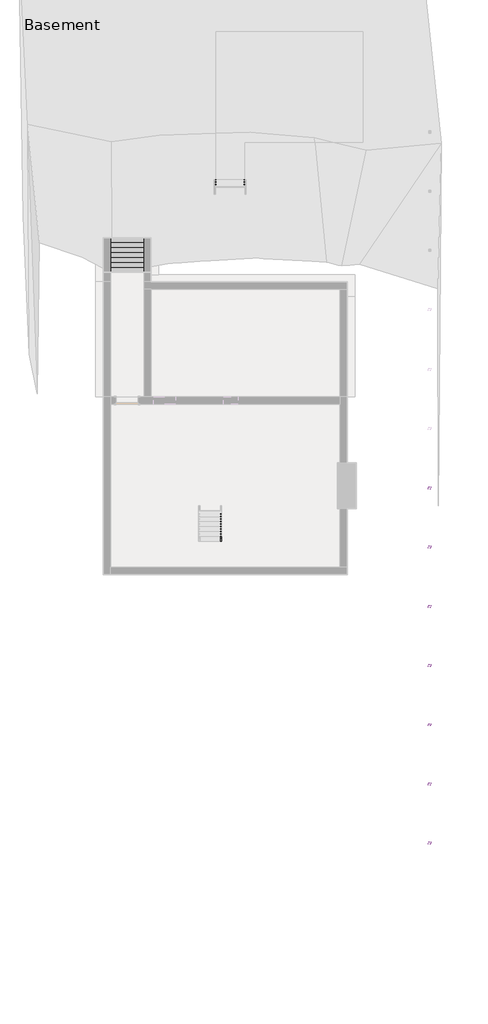
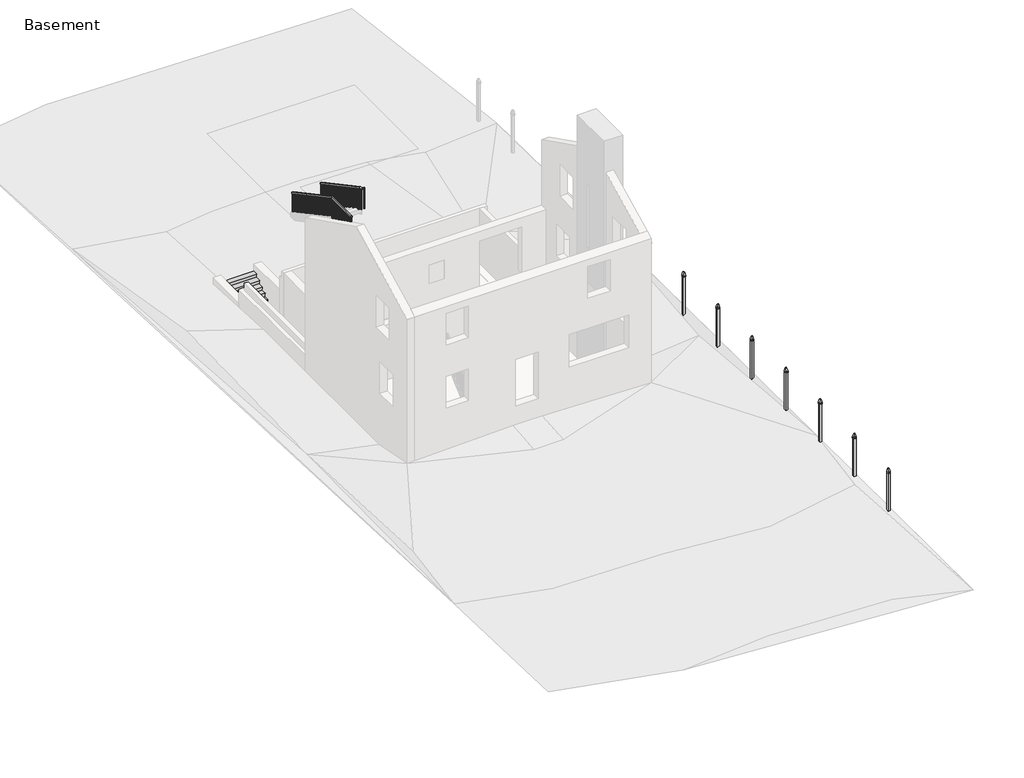
# One storey, part 2 of 3: 7 proxies, 3 railings, 1 stair flight.
"""IFC4 building model written with IfcOpenShell, lengths in millimetres."""

import ifcopenshell
import ifcopenshell.guid

model = None  # the IFC model being written
_history = None  # IfcOwnerHistory: only IFC2X3 demands one
_inside = {}  # id of a spatial element -> (the spatial element, [elements in it])
_under = {}  # id of a project, library or spatial element -> (it, [spatial elements below it])
_declared = {}  # id of a project -> (the project, [libraries it declares])
_typed = {}  # id of a type object -> (the type object, [elements of that type])
_made_of = {}  # id of a material, layer set ... -> (it, [elements and type objects made of it])


def new_model(schema):
    """Start an empty IFC model of exactly this schema.

    Asked for "IFC4X3", IfcOpenShell would pick the latest addendum, in which some entities
    have other attributes; the version numbers below select the first issue.
    IFC2X3 requires an IfcOwnerHistory on every rooted entity: one is made here for all.
    """
    global model, _history
    if schema == "IFC4X3":
        model = ifcopenshell.file(schema_version=(4, 3, 0, 0))
    else:
        model = ifcopenshell.file(schema=schema)
    _inside.clear()
    _under.clear()
    _declared.clear()
    _typed.clear()
    _made_of.clear()
    _history = None
    if model.schema == "IFC2X3":
        org = make("IfcOrganization", Name="unknown")
        user = make(
            "IfcPersonAndOrganization",
            ThePerson=make("IfcPerson", FamilyName="unknown"),
            TheOrganization=org,
        )
        app = make(
            "IfcApplication",
            ApplicationDeveloper=org,
            Version="unknown",
            ApplicationFullName="unknown",
            ApplicationIdentifier="unknown",
        )
        _history = make(
            "IfcOwnerHistory",
            OwningUser=user,
            OwningApplication=app,
            ChangeAction="ADDED",
            CreationDate=0,
        )
    return model


def make(cls, **values):
    """One entity of the class cls with the attributes given. An attribute that is None is left unset."""
    return model.create_entity(
        cls, **{name: value for name, value in values.items() if value is not None}
    )


def rooted(cls, **values):
    """An entity with a GlobalId (a new one), such as an element, a storey or a relation."""
    return make(cls, GlobalId=ifcopenshell.guid.new(), OwnerHistory=_history, **values)


def si_unit(unit_type, name, prefix=None):
    """IfcSIUnit, for example si_unit("LENGTHUNIT", "METRE", prefix="MILLI")."""
    return make("IfcSIUnit", UnitType=unit_type, Prefix=prefix, Name=name)


def assignment(units):
    """IfcUnitAssignment: the units of a project."""
    return None if units is None else make("IfcUnitAssignment", Units=units)


def point(xyz):
    """IfcCartesianPoint."""
    return None if xyz is None else make("IfcCartesianPoint", Coordinates=xyz)


def direction(xyz):
    """IfcDirection."""
    return None if xyz is None else make("IfcDirection", DirectionRatios=xyz)


def frame(location, z_axis=None, x_axis=None):
    """IfcAxis2Placement3D, a coordinate frame: its origin and axes. An axis left out is left unset."""
    return make(
        "IfcAxis2Placement3D",
        Location=point(location),
        Axis=direction(z_axis),
        RefDirection=direction(x_axis),
    )


def origin():
    """The frame at (0, 0, 0) with its axes left unset."""
    return frame((0.0, 0.0, 0.0))


def origin_with_axes():
    """The frame at (0, 0, 0) with the z axis (0, 0, 1) and the x axis (1, 0, 0) written out."""
    return frame((0.0, 0.0, 0.0), z_axis=(0.0, 0.0, 1.0), x_axis=(1.0, 0.0, 0.0))


def place(relative_to, where):
    """IfcLocalPlacement: puts the frame where relative to a parent placement (None: the world)."""
    return make(
        "IfcLocalPlacement", PlacementRelTo=relative_to, RelativePlacement=where
    )


def context(
    kind, dimensions, precision=None, world=None, true_north=None, identifier=None
):
    """IfcGeometricRepresentationContext, for example the 3D "Model" context."""
    return make(
        "IfcGeometricRepresentationContext",
        ContextIdentifier=identifier,
        ContextType=kind,
        CoordinateSpaceDimension=dimensions,
        Precision=precision,
        WorldCoordinateSystem=world,
        TrueNorth=true_north,
    )


def project(units=None, contexts=None):
    """IfcProject with its units and contexts."""
    return rooted(
        "IfcProject",
        Name="project",
        RepresentationContexts=contexts,
        UnitsInContext=assignment(units),
    )


def spatial(cls, under=None, at=None, **own):
    """A site, building, storey or space (cls), placed at a placement, below another one or the project."""
    s = rooted(cls, ObjectPlacement=at, **own)
    if under is not None:
        _under.setdefault(under.id(), (under, []))[1].append(s)
    return s


def polyline(points):
    """IfcPolyline through the points."""
    return make("IfcPolyline", Points=[point(p) for p in points])


def ellipse_curve(where, semi_axis1, semi_axis2):
    """IfcEllipse in the frame where."""
    return make(
        "IfcEllipse", Position=where, SemiAxis1=semi_axis1, SemiAxis2=semi_axis2
    )


def outline(outer, holes=None, kind="AREA"):
    """IfcArbitraryClosedProfileDef: a profile drawn as a closed curve; with holes, ...WithVoids."""
    if holes is None:
        return make("IfcArbitraryClosedProfileDef", ProfileType=kind, OuterCurve=outer)
    return make(
        "IfcArbitraryProfileDefWithVoids",
        ProfileType=kind,
        OuterCurve=outer,
        InnerCurves=holes,
    )


def extrude(swept, where, along, depth):
    """IfcExtrudedAreaSolid: the profile swept, set in the frame where, extruded along a direction by depth."""
    return make(
        "IfcExtrudedAreaSolid",
        SweptArea=swept,
        Position=where,
        ExtrudedDirection=direction(along),
        Depth=depth,
    )


def faces_of(points, faces, orient=None, outer=None):
    """IfcFace entities. A face is a list of loops; a loop is a list of indices into points, from 0.

    orient and outer hold one flag for each loop. By default every Orientation is true, the
    first loop of a face is its IfcFaceOuterBound and the others are IfcFaceBound.
    """
    made = []
    for i, loops in enumerate(faces):
        bounds = []
        for j, loop in enumerate(loops):
            is_outer = j == 0 if outer is None else outer[i][j]
            bounds.append(
                make(
                    "IfcFaceOuterBound" if is_outer else "IfcFaceBound",
                    Bound=make("IfcPolyLoop", Polygon=[points[k] for k in loop]),
                    Orientation=True if orient is None else orient[i][j],
                )
            )
        made.append(make("IfcFace", Bounds=bounds))
    return made


def faceted_brep(points, faces, orient=None, outer=None, voids=None):
    """IfcFacetedBrep: a solid bounded by flat faces; with voids (closed shells), ...WithVoids."""
    shared = [point(p) for p in points]
    hull = make("IfcClosedShell", CfsFaces=faces_of(shared, faces, orient, outer))
    if voids is None:
        return make("IfcFacetedBrep", Outer=hull)
    return make(
        "IfcFacetedBrepWithVoids",
        Outer=hull,
        Voids=[
            make(cls, CfsFaces=faces_of(shared, fs, o, b)) for cls, fs, o, b in voids
        ],
    )


def shape(context_of_items, identifier, shape_type, items):
    """IfcShapeRepresentation: the items that make up one representation, for example the "Body"."""
    return make(
        "IfcShapeRepresentation",
        ContextOfItems=context_of_items,
        RepresentationIdentifier=identifier,
        RepresentationType=shape_type,
        Items=items,
    )


def source(mapping_origin, context_of_items, identifier, shape_type, items):
    """IfcRepresentationMap: a shape defined once, which mapped items show again and again."""
    return make(
        "IfcRepresentationMap",
        MappingOrigin=mapping_origin,
        MappedRepresentation=shape(context_of_items, identifier, shape_type, items),
    )


def transform(
    local_origin,
    x_axis=None,
    y_axis=None,
    z_axis=None,
    scale=None,
    scale2=None,
    scale3=None,
    uniform=True,
):
    """IfcCartesianTransformationOperator3D, or its non-uniform kind. x_axis, y_axis, z_axis: its Axis1, 2, 3."""
    if uniform:
        return make(
            "IfcCartesianTransformationOperator3D",
            Axis1=direction(x_axis),
            Axis2=direction(y_axis),
            LocalOrigin=point(local_origin),
            Scale=scale,
            Axis3=direction(z_axis),
        )
    return make(
        "IfcCartesianTransformationOperator3DnonUniform",
        Axis1=direction(x_axis),
        Axis2=direction(y_axis),
        LocalOrigin=point(local_origin),
        Scale=scale,
        Axis3=direction(z_axis),
        Scale2=scale2,
        Scale3=scale3,
    )


def mapped(mapping_source, mapping_target):
    """IfcMappedItem: shows the shape of a source again, moved by a transform."""
    return make(
        "IfcMappedItem", MappingSource=mapping_source, MappingTarget=mapping_target
    )


def made_of(thing, what):
    """Note that an element or type object is made of a material, layer set ...; save() writes the relation."""
    if what is not None:
        _made_of.setdefault(what.id(), (what, []))[1].append(thing)
    return thing


def element(
    cls,
    number,
    at=None,
    inside=None,
    cuts=None,
    type_object=None,
    material=None,
    context=None,
    identifier="Body",
    shape_type=None,
    held_by="IfcProductDefinitionShape",
    body=None,
    shapes=None,
    **own,
):
    """One element of the class cls, such as IfcWall. Its Tag is "e" and its number.

    at: its placement. inside: the storey or other place that contains it. cuts: it is an
    opening in that element (IfcRelVoidsElement). A single representation is given by context,
    identifier, shape_type and body (its items); several are given by shapes. held_by: the class
    of the entity that holds the representations. save() writes the other relations.
    """
    e = rooted(cls, Tag="e%d" % number, ObjectPlacement=at, **own)
    if body is not None:
        shapes = [shape(context, identifier, shape_type, body)]
    if shapes is not None:
        e.Representation = make(held_by, Representations=shapes)
    if inside is not None:
        _inside.setdefault(inside.id(), (inside, []))[1].append(e)
    if cuts is not None:
        rooted(
            "IfcRelVoidsElement", RelatingBuildingElement=cuts, RelatedOpeningElement=e
        )
    if type_object is not None:
        _typed.setdefault(type_object.id(), (type_object, []))[1].append(e)
    return made_of(e, material)


def aggregate(whole, parts):
    """IfcRelAggregates: a whole, such as a stair, and the parts it consists of."""
    return rooted("IfcRelAggregates", RelatingObject=whole, RelatedObjects=parts)


def save(model, path):
    """Write the relations noted so far, then the file.

    IfcRelAggregates (storeys below a building ...), IfcRelContainedInSpatialStructure (elements
    in a storey), IfcRelDefinesByType, IfcRelAssociatesMaterial and IfcRelDeclares: one each for
    every whole, place, type object, material and project.
    """
    for whole, parts in _under.values():
        aggregate(whole, parts)
    for where, things in _inside.values():
        rooted(
            "IfcRelContainedInSpatialStructure",
            RelatedElements=things,
            RelatingStructure=where,
        )
    for kind, things in _typed.values():
        rooted("IfcRelDefinesByType", RelatedObjects=things, RelatingType=kind)
    for what, things in _made_of.values():
        rooted("IfcRelAssociatesMaterial", RelatedObjects=things, RelatingMaterial=what)
    for by, libraries in _declared.values():
        rooted("IfcRelDeclares", RelatingContext=by, RelatedDefinitions=libraries)
    model.write(path)


def plane_surface(at):
    """IfcPlane: the flat surface through the origin of the frame at, square to its z axis."""
    return make("IfcPlane", Position=at)


def cylinder_surface(at, radius):
    """IfcCylindricalSurface: all points at the distance radius from the z axis of the frame at."""
    return make("IfcCylindricalSurface", Position=at, Radius=radius)


def revolved_surface(curve, axis_point, axis_direction):
    """IfcSurfaceOfRevolution: the curve turned about the line through axis_point along axis_direction."""
    return make(
        "IfcSurfaceOfRevolution",
        SweptCurve=make("IfcArbitraryOpenProfileDef", ProfileType="CURVE", Curve=curve),
        AxisPosition=make("IfcAxis1Placement", Location=point(axis_point), Axis=direction(axis_direction)),
    )


def advanced_brep(points, edges, surfaces, faces):
    """IfcAdvancedBrep: a solid bounded by faces that lie on surfaces and meet in shared edges.

    An edge is (start, end): straight between two places in points (the first is 0);
    or (start, end, curve); or (start, end, curve, False) where it runs against its curve.
    A face is (place in surfaces, loops), or (place, loops, False) where it looks against
    its surface's normal. A loop lists edges by number (the first is 1), with a minus sign
    where the edge is run from its end to its start. The first loop is the outer one.
    """
    corners = [point(p) for p in points]
    vertices = [make("IfcVertexPoint", VertexGeometry=c) for c in corners]
    made = []
    for start, end, *more in edges:
        made.append(
            make(
                "IfcEdgeCurve",
                EdgeStart=vertices[start],
                EdgeEnd=vertices[end],
                EdgeGeometry=more[0] if more else make("IfcPolyline", Points=[corners[start], corners[end]]),
                SameSense=more[1] if len(more) > 1 else True,
            )
        )
    hull = []
    for where, loops, *sense in faces:
        bounds = []
        for j, loop in enumerate(loops):
            ring = [make("IfcOrientedEdge", EdgeElement=made[abs(k) - 1], Orientation=k > 0) for k in loop]
            bounds.append(
                make(
                    "IfcFaceOuterBound" if j == 0 else "IfcFaceBound",
                    Bound=make("IfcEdgeLoop", EdgeList=ring),
                    Orientation=True,
                )
            )
        hull.append(make("IfcAdvancedFace", Bounds=bounds, FaceSurface=surfaces[where], SameSense=sense[0] if sense else True))
    return make("IfcAdvancedBrep", Outer=make("IfcClosedShell", CfsFaces=hull))


def proxy_fa72a640(model_context):
    return source(origin(), model_context, "Body", "SolidModel", [
        extrude(outline(polyline([(44.45, 107.95), (44.45, 19.05), (-44.45, 19.05), (-44.45, 107.95), (44.45, 107.95)])), frame((0.0, 0.0, -228.6), z_axis=(0.0, 0.0, 1.0), x_axis=(1.0, 0.0, 0.0)), (0.0, 0.0, 1.0), 1676.4),
        advanced_brep(
        [(44.45, 19.05, 1428.75), (44.45, 19.05, 1447.8), (44.45, 107.95, 1447.8), (44.45, 107.95, 1428.75), (50.8, 12.7, 1460.5), (50.8, 12.7, 1428.75), (50.8, 114.3, 1428.75), (50.8, 114.3, 1460.5), (-44.45, 107.95, 1447.8), (-44.45, 107.95, 1428.75), (-50.8, 114.3, 1428.75), (-50.8, 114.3, 1460.5), (-44.45, 19.05, 1447.8), (-44.45, 19.05, 1428.75), (-50.8, 12.7, 1428.75), (-50.8, 12.7, 1460.5), (21.7547368, 85.2547368, 1622.5472198), (-21.7547368, 85.2547368, 1622.5472198), (-21.7547368, 41.7452632, 1622.5472198), (21.7547368, 41.7452632, 1622.5472198), (50.8, 114.3, 1485.9), (50.8, 12.7, 1485.9), (-50.8, 114.3, 1485.9), (-50.8, 12.7, 1485.9)],
        [
            (0, 1),
            (1, 2),
            (2, 3),
            (3, 0),
            (4, 5),
            (5, 6),
            (6, 7),
            (7, 4),
            (2, 8),
            (8, 9),
            (9, 3),
            (6, 10),
            (10, 11),
            (11, 7),
            (8, 12),
            (12, 13),
            (13, 9),
            (10, 14),
            (14, 15),
            (15, 11),
            (0, 13),
            (12, 1),
            (5, 14),
            (4, 15),
            (16, 17),
            (17, 18),
            (18, 19),
            (19, 16),
            (7, 20, ellipse_curve(frame((57.3454302, 120.8454302, 1473.2), z_axis=(-0.7071067811865475, 0.7071067811865475, 0.0), x_axis=(0.7071067811865474, 0.7071067811865476, 0.0)), 20.2055763, 14.2875)),
            (20, 21),
            (21, 4, ellipse_curve(frame((57.3454302, 6.1545698, 1473.2), z_axis=(-0.7071067811865475, -0.7071067811865475, 0.0), x_axis=(-0.7071067811865474, 0.7071067811865476, 0.0)), 20.2055763, 14.2875)),
            (19, 21, ellipse_curve(frame((-351.3440328, 414.8440328, 1471.8321377), z_axis=(0.7071067811865475, 0.7071067811865475, 0.0), x_axis=(0.7071067811865474, -0.7071067811865476, 0.0)), 569.065423, 402.3900195)),
            (20, 16, ellipse_curve(frame((-351.3440328, -287.8440328, 1471.8321377), z_axis=(0.7071067811865475, -0.7071067811865475, 0.0), x_axis=(-0.7071067811865474, -0.7071067811865476, 0.0)), 569.065423, 402.3900195)),
            (11, 22, ellipse_curve(frame((-57.3454302, 120.8454302, 1473.2), z_axis=(-0.7071067811865475, -0.7071067811865475, 0.0), x_axis=(-0.7071067811865476, 0.7071067811865474, 0.0)), 20.2055763, 14.2875)),
            (22, 20),
            (22, 17, ellipse_curve(frame((351.3440328, -287.8440328, 1471.8321377), z_axis=(0.7071067811865475, 0.7071067811865475, 0.0), x_axis=(0.7071067811865476, -0.7071067811865474, 0.0)), 569.065423, 402.3900195)),
            (15, 23, ellipse_curve(frame((-57.3454302, 6.1545698, 1473.2), z_axis=(0.7071067811865475, -0.7071067811865475, 0.0), x_axis=(-0.7071067811865474, -0.7071067811865476, 0.0)), 20.2055763, 14.2875)),
            (23, 22),
            (23, 18, ellipse_curve(frame((351.3440328, 414.8440328, 1471.8321377), z_axis=(-0.7071067811865475, 0.7071067811865475, 0.0), x_axis=(0.7071067811865474, 0.7071067811865476, 0.0)), 569.065423, 402.3900195)),
            (21, 23),
        ],
        [
            plane_surface(frame((44.45, 19.05, 1447.8), z_axis=(-1.0, 0.0, 0.0), x_axis=(0.0, 1.0, 0.0))),
            plane_surface(frame((50.8, 12.7, 1428.75), z_axis=(1.0, 0.0, 0.0), x_axis=(0.0, 1.0, 0.0))),
            plane_surface(frame((44.45, 107.95, 1447.8), z_axis=(0.0, -1.0, 0.0), x_axis=(-1.0, 0.0, 0.0))),
            plane_surface(frame((50.8, 114.3, 1428.75), z_axis=(0.0, 1.0, 0.0), x_axis=(-1.0, 0.0, 0.0))),
            plane_surface(frame((-44.45, 107.95, 1447.8), z_axis=(1.0, 0.0, 0.0), x_axis=(0.0, -1.0, 0.0))),
            plane_surface(frame((-50.8, 114.3, 1428.75), z_axis=(-1.0, 0.0, 0.0), x_axis=(0.0, -1.0, 0.0))),
            plane_surface(frame((-44.45, 19.05, 1447.8), z_axis=(0.0, 1.0, 0.0), x_axis=(1.0, 0.0, 0.0))),
            plane_surface(frame((-15.4047368, 48.0952632, 1447.8), z_axis=(0.0, 0.0, -1.0), x_axis=(1.0, 0.0, 0.0))),
            plane_surface(frame((-44.45, 19.05, 1428.75), z_axis=(0.0, 0.0, -1.0), x_axis=(1.0, 0.0, 0.0))),
            plane_surface(frame((-50.8, 12.7, 1428.75), z_axis=(0.0, -1.0, 0.0), x_axis=(1.0, 0.0, 0.0))),
            plane_surface(frame((-21.7547368, 41.7452632, 1622.5472198), z_axis=(0.0, 0.0, 1.0), x_axis=(1.0, 0.0, 0.0))),
            revolved_surface(polyline([(43.0579302, 135.1329302195122, 1473.2), (43.0579302, -8.132930219512193, 1473.2)]), (57.3454302, 19.05, 1473.2), (0.0, 1.0, 0.0)),
            cylinder_surface(frame((-351.3440328, 19.05, 1471.8321377), z_axis=(0.0, -1.0, 0.0), x_axis=(-1.0, 0.0, 0.0)), 402.3900195),
            revolved_surface(polyline([(-71.63293021951219, 106.5579302, 1473.2), (71.63293021951219, 106.5579302, 1473.2)]), (44.45, 120.8454302, 1473.2), (-1.0, 0.0, 0.0)),
            cylinder_surface(frame((44.45, -287.8440328, 1471.8321377), z_axis=(1.0, 0.0, 0.0), x_axis=(0.0, -1.0, 0.0)), 402.3900195),
            revolved_surface(polyline([(-43.0579302, -8.13293021951219, 1473.2), (-43.0579302, 135.1329302195122, 1473.2)]), (-57.3454302, 107.95, 1473.2), (0.0, -1.0, 0.0)),
            cylinder_surface(frame((351.3440328, 107.95, 1471.8321377), z_axis=(0.0, 1.0, 0.0), x_axis=(1.0, 0.0, 0.0)), 402.3900195),
            revolved_surface(polyline([(71.63293021951218, 20.4420698, 1473.2), (-71.63293021951219, 20.4420698, 1473.2)]), (-44.45, 6.1545698, 1473.2), (1.0, 0.0, 0.0)),
            cylinder_surface(frame((-44.45, 414.8440328, 1471.8321377), z_axis=(-1.0, 0.0, 0.0), x_axis=(0.0, 1.0, 0.0)), 402.3900195),
        ],
        [
            (0, [[1, 2, 3, 4]]),
            (1, [[5, 6, 7, 8]]),
            (2, [[-3, 9, 10, 11]]),
            (3, [[-7, 12, 13, 14]]),
            (4, [[-10, 15, 16, 17]]),
            (5, [[-13, 18, 19, 20]]),
            (6, [[-1, 21, -16, 22]]),
            (7, [[-2, -22, -15, -9]]),
            (8, [[-6, 23, -18, -12], [-4, -11, -17, -21]]),
            (9, [[-5, 24, -19, -23]]),
            (10, [[25, 26, 27, 28]]),
            (11, [[-8, 29, 30, 31]]),
            (12, [[-28, 32, -30, 33]]),
            (13, [[-14, 34, 35, -29]]),
            (14, [[-25, -33, -35, 36]]),
            (15, [[-20, 37, 38, -34]]),
            (16, [[-26, -36, -38, 39]]),
            (17, [[-24, -31, 40, -37]]),
            (18, [[-27, -39, -40, -32]]),
        ],
    ),
    ])


model = new_model("IFC4")

# Units and contexts
model_context = context("Model", 3, world=origin())
ifc_project = project(units=[si_unit("LENGTHUNIT", "METRE", prefix="MILLI")], contexts=[model_context])

# Site, building, storey
site = spatial("IfcSite", under=ifc_project)
building = spatial("IfcBuilding", under=site)
storey = spatial("IfcBuildingStorey", under=building, Name="Basement", Elevation=-2667.0)

# Proxies
placement = place(None, origin())
proxy_shape = proxy_fa72a640(model_context)
element("IfcBuildingElementProxy", 1, Name="SUP_Post : 4\" x 4\"", ObjectType="SUP_Post : 4\" x 4\"", at=placement, inside=storey, context=model_context, shape_type="MappedRepresentation", body=[
    mapped(proxy_shape, transform((7523.8891925, -597.8195486, -1086.34775), x_axis=(0.0, 1.0, 0.0), y_axis=(-1.0, 0.0, 0.0), z_axis=(0.0, 0.0, 1.0))),
])
element("IfcBuildingElementProxy", 2, Name="SUP_Post : 4\" x 4\"", ObjectType="SUP_Post : 4\" x 4\"", at=placement, inside=storey, context=model_context, shape_type="MappedRepresentation", body=[
    mapped(proxy_shape, transform((7523.8891925, -3034.8101148, -1003.4529933), x_axis=(0.0, 1.0, 0.0), y_axis=(-1.0, 0.0, 0.0), z_axis=(0.0, 0.0, 1.0))),
])
element("IfcBuildingElementProxy", 3, Name="SUP_Post : 4\" x 4\"", ObjectType="SUP_Post : 4\" x 4\"", at=placement, inside=storey, context=model_context, shape_type="MappedRepresentation", body=[
    mapped(proxy_shape, transform((7523.8891925, -5471.8006809, -920.5582365), x_axis=(0.0, 1.0, 0.0), y_axis=(-1.0, 0.0, 0.0), z_axis=(0.0, 0.0, 1.0))),
])
element("IfcBuildingElementProxy", 4, Name="SUP_Post : 4\" x 4\"", ObjectType="SUP_Post : 4\" x 4\"", at=placement, inside=storey, context=model_context, shape_type="MappedRepresentation", body=[
    mapped(proxy_shape, transform((7523.8891925, -7908.3149466, -826.7906503), x_axis=(0.0, 1.0, 0.0), y_axis=(-1.0, 0.0, 0.0), z_axis=(0.0, 0.0, 1.0))),
])
element("IfcBuildingElementProxy", 5, Name="SUP_Post : 4\" x 4\"", ObjectType="SUP_Post : 4\" x 4\"", at=placement, inside=storey, context=model_context, shape_type="MappedRepresentation", body=[
    mapped(proxy_shape, transform((7523.8891925, -10343.9591395, -723.8999758), x_axis=(0.0, 1.0, 0.0), y_axis=(-1.0, 0.0, 0.0), z_axis=(0.0, 0.0, 1.0))),
])
element("IfcBuildingElementProxy", 6, Name="SUP_Post : 4\" x 4\"", ObjectType="SUP_Post : 4\" x 4\"", at=placement, inside=storey, context=model_context, shape_type="MappedRepresentation", body=[
    mapped(proxy_shape, transform((7523.8891925, -12782.1972588, -749.7426083), x_axis=(0.0, 1.0, 0.0), y_axis=(-1.0, 0.0, 0.0), z_axis=(0.0, 0.0, 1.0))),
])
element("IfcBuildingElementProxy", 7, Name="SUP_Post : 4\" x 4\"", ObjectType="SUP_Post : 4\" x 4\"", at=placement, inside=storey, context=model_context, shape_type="MappedRepresentation", body=[
    mapped(proxy_shape, transform((7523.8891925, -15220.4059061, -780.2901471), x_axis=(0.0, 1.0, 0.0), y_axis=(-1.0, 0.0, 0.0), z_axis=(0.0, 0.0, 1.0))),
])

# Railings
element("IfcRailing", 8, ObjectType="Handrail - Rectangular", at=placement, inside=storey, context=model_context, shape_type="SweptSolid", body=[
    extrude(outline(polyline([(-2791.5111242, -1631.7331862), (-2791.5111242, -1562.1), (-149.9111242, 914.4), (-149.9111242, 844.7668138), (-2791.5111242, -1631.7331862)])), frame((-1163.1803068, 0.0, 0.0), z_axis=(1.0, 0.0, 0.0), x_axis=(0.0, 1.0, 0.0)), (0.0, 0.0, 1.0), 50.8),
    extrude(outline(polyline([(-261.0361242, 740.5871263), (-241.9861242, 758.4465013), (-241.9861242, -190.5), (-261.0361242, -190.5), (-261.0361242, 740.5871263)])), frame((-1147.3053068, 0.0, 0.0), z_axis=(1.0, 0.0, 0.0), x_axis=(0.0, 1.0, 0.0)), (0.0, 0.0, 1.0), 19.05),
    extrude(outline(polyline([(-362.6361242, 645.3371263), (-343.5861242, 663.1965013), (-343.5861242, -190.5), (-362.6361242, -190.5), (-362.6361242, 645.3371263)])), frame((-1147.3053068, 0.0, 0.0), z_axis=(1.0, 0.0, 0.0), x_axis=(0.0, 1.0, 0.0)), (0.0, 0.0, 1.0), 19.05),
    extrude(outline(polyline([(-464.2361242, 550.0871263), (-445.1861242, 567.9465013), (-445.1861242, -381.0), (-464.2361242, -381.0), (-464.2361242, 550.0871263)])), frame((-1147.3053068, 0.0, 0.0), z_axis=(1.0, 0.0, 0.0), x_axis=(0.0, 1.0, 0.0)), (0.0, 0.0, 1.0), 19.05),
    extrude(outline(polyline([(-565.8361242, 454.8371263), (-546.7861242, 472.6965013), (-546.7861242, -381.0), (-565.8361242, -381.0), (-565.8361242, 454.8371263)])), frame((-1147.3053068, 0.0, 0.0), z_axis=(1.0, 0.0, 0.0), x_axis=(0.0, 1.0, 0.0)), (0.0, 0.0, 1.0), 19.05),
    extrude(outline(polyline([(-667.4361242, 359.5871263), (-648.3861242, 377.4465013), (-648.3861242, -571.5), (-667.4361242, -571.5), (-667.4361242, 359.5871263)])), frame((-1147.3053068, 0.0, 0.0), z_axis=(1.0, 0.0, 0.0), x_axis=(0.0, 1.0, 0.0)), (0.0, 0.0, 1.0), 19.05),
    extrude(outline(polyline([(-769.0361242, 264.3371263), (-749.9861242, 282.1965013), (-749.9861242, -571.5), (-769.0361242, -571.5), (-769.0361242, 264.3371263)])), frame((-1147.3053068, 0.0, 0.0), z_axis=(1.0, 0.0, 0.0), x_axis=(0.0, 1.0, 0.0)), (0.0, 0.0, 1.0), 19.05),
    extrude(outline(polyline([(-870.6361242, 169.0871263), (-851.5861242, 186.9465013), (-851.5861242, -762.0), (-870.6361242, -762.0), (-870.6361242, 169.0871263)])), frame((-1147.3053068, 0.0, 0.0), z_axis=(1.0, 0.0, 0.0), x_axis=(0.0, 1.0, 0.0)), (0.0, 0.0, 1.0), 19.05),
    extrude(outline(polyline([(-972.2361242, 73.8371263), (-953.1861242, 91.6965013), (-953.1861242, -762.0), (-972.2361242, -762.0), (-972.2361242, 73.8371263)])), frame((-1147.3053068, 0.0, 0.0), z_axis=(1.0, 0.0, 0.0), x_axis=(0.0, 1.0, 0.0)), (0.0, 0.0, 1.0), 19.05),
    extrude(outline(polyline([(-1073.8361242, -21.4128737), (-1054.7861242, -3.5534987), (-1054.7861242, -952.5), (-1073.8361242, -952.5), (-1073.8361242, -21.4128737)])), frame((-1147.3053068, 0.0, 0.0), z_axis=(1.0, 0.0, 0.0), x_axis=(0.0, 1.0, 0.0)), (0.0, 0.0, 1.0), 19.05),
    extrude(outline(polyline([(-1175.4361242, -116.6628737), (-1156.3861242, -98.8034987), (-1156.3861242, -952.5), (-1175.4361242, -952.5), (-1175.4361242, -116.6628737)])), frame((-1147.3053068, 0.0, 0.0), z_axis=(1.0, 0.0, 0.0), x_axis=(0.0, 1.0, 0.0)), (0.0, 0.0, 1.0), 19.05),
    extrude(outline(polyline([(-1277.0361242, -211.9128737), (-1257.9861242, -194.0534987), (-1257.9861242, -1143.0), (-1277.0361242, -1143.0), (-1277.0361242, -211.9128737)])), frame((-1147.3053068, 0.0, 0.0), z_axis=(1.0, 0.0, 0.0), x_axis=(0.0, 1.0, 0.0)), (0.0, 0.0, 1.0), 19.05),
    extrude(outline(polyline([(-1378.6361242, -307.1628737), (-1359.5861242, -289.3034987), (-1359.5861242, -1143.0), (-1378.6361242, -1143.0), (-1378.6361242, -307.1628737)])), frame((-1147.3053068, 0.0, 0.0), z_axis=(1.0, 0.0, 0.0), x_axis=(0.0, 1.0, 0.0)), (0.0, 0.0, 1.0), 19.05),
    extrude(outline(polyline([(-1480.2361242, -402.4128737), (-1461.1861242, -384.5534987), (-1461.1861242, -1333.5), (-1480.2361242, -1333.5), (-1480.2361242, -402.4128737)])), frame((-1147.3053068, 0.0, 0.0), z_axis=(1.0, 0.0, 0.0), x_axis=(0.0, 1.0, 0.0)), (0.0, 0.0, 1.0), 19.05),
    extrude(outline(polyline([(-1581.8361242, -497.6628737), (-1562.7861242, -479.8034987), (-1562.7861242, -1333.5), (-1581.8361242, -1333.5), (-1581.8361242, -497.6628737)])), frame((-1147.3053068, 0.0, 0.0), z_axis=(1.0, 0.0, 0.0), x_axis=(0.0, 1.0, 0.0)), (0.0, 0.0, 1.0), 19.05),
    extrude(outline(polyline([(-1683.4361242, -592.9128737), (-1664.3861242, -575.0534987), (-1664.3861242, -1524.0), (-1683.4361242, -1524.0), (-1683.4361242, -592.9128737)])), frame((-1147.3053068, 0.0, 0.0), z_axis=(1.0, 0.0, 0.0), x_axis=(0.0, 1.0, 0.0)), (0.0, 0.0, 1.0), 19.05),
    extrude(outline(polyline([(-1785.0361242, -688.1628737), (-1765.9861242, -670.3034987), (-1765.9861242, -1524.0), (-1785.0361242, -1524.0), (-1785.0361242, -688.1628737)])), frame((-1147.3053068, 0.0, 0.0), z_axis=(1.0, 0.0, 0.0), x_axis=(0.0, 1.0, 0.0)), (0.0, 0.0, 1.0), 19.05),
    extrude(outline(polyline([(-1886.6361242, -783.4128737), (-1867.5861242, -765.5534987), (-1867.5861242, -1714.5), (-1886.6361242, -1714.5), (-1886.6361242, -783.4128737)])), frame((-1147.3053068, 0.0, 0.0), z_axis=(1.0, 0.0, 0.0), x_axis=(0.0, 1.0, 0.0)), (0.0, 0.0, 1.0), 19.05),
    extrude(outline(polyline([(-1988.2361242, -878.6628737), (-1969.1861242, -860.8034987), (-1969.1861242, -1714.5), (-1988.2361242, -1714.5), (-1988.2361242, -878.6628737)])), frame((-1147.3053068, 0.0, 0.0), z_axis=(1.0, 0.0, 0.0), x_axis=(0.0, 1.0, 0.0)), (0.0, 0.0, 1.0), 19.05),
    extrude(outline(polyline([(-2089.8361242, -973.9128737), (-2070.7861242, -956.0534987), (-2070.7861242, -1905.0), (-2089.8361242, -1905.0), (-2089.8361242, -973.9128737)])), frame((-1147.3053068, 0.0, 0.0), z_axis=(1.0, 0.0, 0.0), x_axis=(0.0, 1.0, 0.0)), (0.0, 0.0, 1.0), 19.05),
    extrude(outline(polyline([(-2191.4361242, -1069.1628737), (-2172.3861242, -1051.3034987), (-2172.3861242, -1905.0), (-2191.4361242, -1905.0), (-2191.4361242, -1069.1628737)])), frame((-1147.3053068, 0.0, 0.0), z_axis=(1.0, 0.0, 0.0), x_axis=(0.0, 1.0, 0.0)), (0.0, 0.0, 1.0), 19.05),
    extrude(outline(polyline([(-2293.0361242, -1164.4128737), (-2273.9861242, -1146.5534987), (-2273.9861242, -2095.5), (-2293.0361242, -2095.5), (-2293.0361242, -1164.4128737)])), frame((-1147.3053068, 0.0, 0.0), z_axis=(1.0, 0.0, 0.0), x_axis=(0.0, 1.0, 0.0)), (0.0, 0.0, 1.0), 19.05),
    extrude(outline(polyline([(-2394.6361242, -1259.6628737), (-2375.5861242, -1241.8034987), (-2375.5861242, -2095.5), (-2394.6361242, -2095.5), (-2394.6361242, -1259.6628737)])), frame((-1147.3053068, 0.0, 0.0), z_axis=(1.0, 0.0, 0.0), x_axis=(0.0, 1.0, 0.0)), (0.0, 0.0, 1.0), 19.05),
    extrude(outline(polyline([(-2496.2361242, -1354.9128737), (-2477.1861242, -1337.0534987), (-2477.1861242, -2286.0), (-2496.2361242, -2286.0), (-2496.2361242, -1354.9128737)])), frame((-1147.3053068, 0.0, 0.0), z_axis=(1.0, 0.0, 0.0), x_axis=(0.0, 1.0, 0.0)), (0.0, 0.0, 1.0), 19.05),
    extrude(outline(polyline([(-2597.8361242, -1450.1628737), (-2578.7861242, -1432.3034987), (-2578.7861242, -2286.0), (-2597.8361242, -2286.0), (-2597.8361242, -1450.1628737)])), frame((-1147.3053068, 0.0, 0.0), z_axis=(1.0, 0.0, 0.0), x_axis=(0.0, 1.0, 0.0)), (0.0, 0.0, 1.0), 19.05),
    extrude(outline(polyline([(-2699.4361242, -1545.4128737), (-2680.3861242, -1527.5534987), (-2680.3861242, -2476.5), (-2699.4361242, -2476.5), (-2699.4361242, -1545.4128737)])), frame((-1147.3053068, 0.0, 0.0), z_axis=(1.0, 0.0, 0.0), x_axis=(0.0, 1.0, 0.0)), (0.0, 0.0, 1.0), 19.05),
    extrude(outline(polyline([(-168.9611242, 826.9074388), (-149.9111242, 844.7668138), (-149.9111242, -190.5), (-168.9611242, -190.5), (-168.9611242, 826.9074388)])), frame((-1147.3053068, 0.0, 0.0), z_axis=(1.0, 0.0, 0.0), x_axis=(0.0, 1.0, 0.0)), (0.0, 0.0, 1.0), 19.05),
    extrude(outline(polyline([(-2791.5111242, -1631.7331862), (-2772.4611242, -1613.8738112), (-2772.4611242, -2476.5), (-2791.5111242, -2476.5), (-2791.5111242, -1631.7331862)])), frame((-1147.3053068, 0.0, 0.0), z_axis=(1.0, 0.0, 0.0), x_axis=(0.0, 1.0, 0.0)), (0.0, 0.0, 1.0), 19.05),
])
element("IfcRailing", 9, ObjectType="Handrail - Rectangular", at=placement, inside=storey, context=model_context, shape_type="SolidModel", body=[
    faceted_brep([(-1315.5803068, 12092.8888758, -586.5090909), (-1315.5803068, 12092.8888758, -644.1748824), (-1366.3803068, 12092.8888758, -644.1748824), (-1366.3803068, 12092.8888758, -586.5090909), (-1315.5803068, 9298.8888758, 914.4), (-1315.5803068, 9286.107941, 863.6), (-1366.3803068, 9286.107941, 863.6), (-1366.3803068, 9298.8888758, 914.4), (-1315.5803068, 7876.4888758, 914.4), (-1366.3803068, 7876.4888758, 914.4), (-1366.3803068, 7876.4888758, 863.6), (-1315.5803068, 7876.4888758, 863.6)], [[[0, 1, 2, 3]], [[1, 0, 4, 5]], [[2, 1, 5, 6]], [[3, 2, 6, 7]], [[0, 3, 7, 4]], [[8, 9, 10, 11]], [[5, 4, 8, 11]], [[6, 5, 11, 10]], [[7, 6, 10, 9]], [[4, 7, 9, 8]]]),
    extrude(outline(polyline([(-1350.5053068, 7987.6138758), (-1331.4553068, 7987.6138758), (-1331.4553068, 7968.5638758), (-1350.5053068, 7968.5638758), (-1350.5053068, 7987.6138758)])), origin_with_axes(), (0.0, 0.0, 1.0), 863.6),
    extrude(outline(polyline([(-1350.5053068, 8089.2138758), (-1331.4553068, 8089.2138758), (-1331.4553068, 8070.1638758), (-1350.5053068, 8070.1638758), (-1350.5053068, 8089.2138758)])), origin_with_axes(), (0.0, 0.0, 1.0), 863.6),
    extrude(outline(polyline([(-1350.5053068, 8190.8138758), (-1331.4553068, 8190.8138758), (-1331.4553068, 8171.7638758), (-1350.5053068, 8171.7638758), (-1350.5053068, 8190.8138758)])), origin_with_axes(), (0.0, 0.0, 1.0), 863.6),
    extrude(outline(polyline([(-1350.5053068, 8292.4138758), (-1331.4553068, 8292.4138758), (-1331.4553068, 8273.3638758), (-1350.5053068, 8273.3638758), (-1350.5053068, 8292.4138758)])), origin_with_axes(), (0.0, 0.0, 1.0), 863.6),
    extrude(outline(polyline([(-1350.5053068, 8394.0138758), (-1331.4553068, 8394.0138758), (-1331.4553068, 8374.9638758), (-1350.5053068, 8374.9638758), (-1350.5053068, 8394.0138758)])), origin_with_axes(), (0.0, 0.0, 1.0), 863.6),
    extrude(outline(polyline([(-1350.5053068, 8495.6138758), (-1331.4553068, 8495.6138758), (-1331.4553068, 8476.5638758), (-1350.5053068, 8476.5638758), (-1350.5053068, 8495.6138758)])), origin_with_axes(), (0.0, 0.0, 1.0), 863.6),
    extrude(outline(polyline([(-1350.5053068, 8597.2138758), (-1331.4553068, 8597.2138758), (-1331.4553068, 8578.1638758), (-1350.5053068, 8578.1638758), (-1350.5053068, 8597.2138758)])), origin_with_axes(), (0.0, 0.0, 1.0), 863.6),
    extrude(outline(polyline([(-1350.5053068, 8698.8138758), (-1331.4553068, 8698.8138758), (-1331.4553068, 8679.7638758), (-1350.5053068, 8679.7638758), (-1350.5053068, 8698.8138758)])), origin_with_axes(), (0.0, 0.0, 1.0), 863.6),
    extrude(outline(polyline([(-1350.5053068, 8800.4138758), (-1331.4553068, 8800.4138758), (-1331.4553068, 8781.3638758), (-1350.5053068, 8781.3638758), (-1350.5053068, 8800.4138758)])), origin_with_axes(), (0.0, 0.0, 1.0), 863.6),
    extrude(outline(polyline([(-1350.5053068, 8902.0138758), (-1331.4553068, 8902.0138758), (-1331.4553068, 8882.9638758), (-1350.5053068, 8882.9638758), (-1350.5053068, 8902.0138758)])), origin_with_axes(), (0.0, 0.0, 1.0), 863.6),
    extrude(outline(polyline([(-1350.5053068, 9003.6138758), (-1331.4553068, 9003.6138758), (-1331.4553068, 8984.5638758), (-1350.5053068, 8984.5638758), (-1350.5053068, 9003.6138758)])), origin_with_axes(), (0.0, 0.0, 1.0), 863.6),
    extrude(outline(polyline([(-1350.5053068, 9105.2138758), (-1331.4553068, 9105.2138758), (-1331.4553068, 9086.1638758), (-1350.5053068, 9086.1638758), (-1350.5053068, 9105.2138758)])), origin_with_axes(), (0.0, 0.0, 1.0), 863.6),
    extrude(outline(polyline([(-1350.5053068, 9206.8138758), (-1331.4553068, 9206.8138758), (-1331.4553068, 9187.7638758), (-1350.5053068, 9187.7638758), (-1350.5053068, 9206.8138758)])), origin_with_axes(), (0.0, 0.0, 1.0), 863.6),
    extrude(outline(polyline([(9340.1638758, 834.5616879), (9359.2138758, 824.3282168), (9359.2138758, -150.0909091), (9340.1638758, -150.0909091), (9340.1638758, 834.5616879)])), frame((-1350.5053068, 0.0, 0.0), z_axis=(1.0, 0.0, 0.0), x_axis=(0.0, 1.0, 0.0)), (0.0, 0.0, 1.0), 19.05),
    extrude(outline(polyline([(9441.7638758, 779.9831755), (9460.8138758, 769.7497044), (9460.8138758, -150.0909091), (9441.7638758, -150.0909091), (9441.7638758, 779.9831755)])), frame((-1350.5053068, 0.0, 0.0), z_axis=(1.0, 0.0, 0.0), x_axis=(0.0, 1.0, 0.0)), (0.0, 0.0, 1.0), 19.05),
    extrude(outline(polyline([(9543.3638758, 725.4046631), (9562.4138758, 715.171192), (9562.4138758, -150.0909091), (9543.3638758, -150.0909091), (9543.3638758, 725.4046631)])), frame((-1350.5053068, 0.0, 0.0), z_axis=(1.0, 0.0, 0.0), x_axis=(0.0, 1.0, 0.0)), (0.0, 0.0, 1.0), 19.05),
    extrude(outline(polyline([(9644.9638758, 670.8261507), (9664.0138758, 660.5926796), (9664.0138758, -300.1818182), (9644.9638758, -300.1818182), (9644.9638758, 670.8261507)])), frame((-1350.5053068, 0.0, 0.0), z_axis=(1.0, 0.0, 0.0), x_axis=(0.0, 1.0, 0.0)), (0.0, 0.0, 1.0), 19.05),
    extrude(outline(polyline([(9746.5638758, 616.2476383), (9765.6138758, 606.0141672), (9765.6138758, -300.1818182), (9746.5638758, -300.1818182), (9746.5638758, 616.2476383)])), frame((-1350.5053068, 0.0, 0.0), z_axis=(1.0, 0.0, 0.0), x_axis=(0.0, 1.0, 0.0)), (0.0, 0.0, 1.0), 19.05),
    extrude(outline(polyline([(9848.1638758, 561.6691259), (9867.2138758, 551.4356548), (9867.2138758, -300.1818182), (9848.1638758, -300.1818182), (9848.1638758, 561.6691259)])), frame((-1350.5053068, 0.0, 0.0), z_axis=(1.0, 0.0, 0.0), x_axis=(0.0, 1.0, 0.0)), (0.0, 0.0, 1.0), 19.05),
    extrude(outline(polyline([(9949.7638758, 507.0906135), (9968.8138758, 496.8571424), (9968.8138758, -450.2727273), (9949.7638758, -450.2727273), (9949.7638758, 507.0906135)])), frame((-1350.5053068, 0.0, 0.0), z_axis=(1.0, 0.0, 0.0), x_axis=(0.0, 1.0, 0.0)), (0.0, 0.0, 1.0), 19.05),
    extrude(outline(polyline([(10051.3638758, 452.5121011), (10070.4138758, 442.27863), (10070.4138758, -450.2727273), (10051.3638758, -450.2727273), (10051.3638758, 452.5121011)])), frame((-1350.5053068, 0.0, 0.0), z_axis=(1.0, 0.0, 0.0), x_axis=(0.0, 1.0, 0.0)), (0.0, 0.0, 1.0), 19.05),
    extrude(outline(polyline([(10152.9638758, 397.9335887), (10172.0138758, 387.7001176), (10172.0138758, -600.3636364), (10152.9638758, -600.3636364), (10152.9638758, 397.9335887)])), frame((-1350.5053068, 0.0, 0.0), z_axis=(1.0, 0.0, 0.0), x_axis=(0.0, 1.0, 0.0)), (0.0, 0.0, 1.0), 19.05),
    extrude(outline(polyline([(10254.5638758, 343.3550763), (10273.6138758, 333.1216052), (10273.6138758, -600.3636364), (10254.5638758, -600.3636364), (10254.5638758, 343.3550763)])), frame((-1350.5053068, 0.0, 0.0), z_axis=(1.0, 0.0, 0.0), x_axis=(0.0, 1.0, 0.0)), (0.0, 0.0, 1.0), 19.05),
    extrude(outline(polyline([(10356.1638758, 288.7765639), (10375.2138758, 278.5430928), (10375.2138758, -600.3636364), (10356.1638758, -600.3636364), (10356.1638758, 288.7765639)])), frame((-1350.5053068, 0.0, 0.0), z_axis=(1.0, 0.0, 0.0), x_axis=(0.0, 1.0, 0.0)), (0.0, 0.0, 1.0), 19.05),
    extrude(outline(polyline([(10457.7638758, 234.1980515), (10476.8138758, 223.9645804), (10476.8138758, -750.4545455), (10457.7638758, -750.4545455), (10457.7638758, 234.1980515)])), frame((-1350.5053068, 0.0, 0.0), z_axis=(1.0, 0.0, 0.0), x_axis=(0.0, 1.0, 0.0)), (0.0, 0.0, 1.0), 19.05),
    extrude(outline(polyline([(10559.3638758, 179.6195391), (10578.4138758, 169.3860681), (10578.4138758, -750.4545455), (10559.3638758, -750.4545455), (10559.3638758, 179.6195391)])), frame((-1350.5053068, 0.0, 0.0), z_axis=(1.0, 0.0, 0.0), x_axis=(0.0, 1.0, 0.0)), (0.0, 0.0, 1.0), 19.05),
    extrude(outline(polyline([(10660.9638758, 125.0410267), (10680.0138758, 114.8075557), (10680.0138758, -750.4545455), (10660.9638758, -750.4545455), (10660.9638758, 125.0410267)])), frame((-1350.5053068, 0.0, 0.0), z_axis=(1.0, 0.0, 0.0), x_axis=(0.0, 1.0, 0.0)), (0.0, 0.0, 1.0), 19.05),
    extrude(outline(polyline([(10762.5638758, 70.4625143), (10781.6138758, 60.2290433), (10781.6138758, -900.5454545), (10762.5638758, -900.5454545), (10762.5638758, 70.4625143)])), frame((-1350.5053068, 0.0, 0.0), z_axis=(1.0, 0.0, 0.0), x_axis=(0.0, 1.0, 0.0)), (0.0, 0.0, 1.0), 19.05),
    extrude(outline(polyline([(10864.1638758, 15.8840019), (10883.2138758, 5.6505309), (10883.2138758, -900.5454545), (10864.1638758, -900.5454545), (10864.1638758, 15.8840019)])), frame((-1350.5053068, 0.0, 0.0), z_axis=(1.0, 0.0, 0.0), x_axis=(0.0, 1.0, 0.0)), (0.0, 0.0, 1.0), 19.05),
    extrude(outline(polyline([(10965.7638758, -38.6945105), (10984.8138758, -48.9279815), (10984.8138758, -900.5454545), (10965.7638758, -900.5454545), (10965.7638758, -38.6945105)])), frame((-1350.5053068, 0.0, 0.0), z_axis=(1.0, 0.0, 0.0), x_axis=(0.0, 1.0, 0.0)), (0.0, 0.0, 1.0), 19.05),
    extrude(outline(polyline([(11067.3638758, -93.2730229), (11086.4138758, -103.5064939), (11086.4138758, -1050.6363636), (11067.3638758, -1050.6363636), (11067.3638758, -93.2730229)])), frame((-1350.5053068, 0.0, 0.0), z_axis=(1.0, 0.0, 0.0), x_axis=(0.0, 1.0, 0.0)), (0.0, 0.0, 1.0), 19.05),
    extrude(outline(polyline([(11168.9638758, -147.8515353), (11188.0138758, -158.0850063), (11188.0138758, -1050.6363636), (11168.9638758, -1050.6363636), (11168.9638758, -147.8515353)])), frame((-1350.5053068, 0.0, 0.0), z_axis=(1.0, 0.0, 0.0), x_axis=(0.0, 1.0, 0.0)), (0.0, 0.0, 1.0), 19.05),
    extrude(outline(polyline([(11270.5638758, -202.4300477), (11289.6138758, -212.6635187), (11289.6138758, -1200.7272727), (11270.5638758, -1200.7272727), (11270.5638758, -202.4300477)])), frame((-1350.5053068, 0.0, 0.0), z_axis=(1.0, 0.0, 0.0), x_axis=(0.0, 1.0, 0.0)), (0.0, 0.0, 1.0), 19.05),
    extrude(outline(polyline([(11372.1638758, -257.00856), (11391.2138758, -267.2420311), (11391.2138758, -1200.7272727), (11372.1638758, -1200.7272727), (11372.1638758, -257.00856)])), frame((-1350.5053068, 0.0, 0.0), z_axis=(1.0, 0.0, 0.0), x_axis=(0.0, 1.0, 0.0)), (0.0, 0.0, 1.0), 19.05),
    extrude(outline(polyline([(11473.7638758, -311.5870724), (11492.8138758, -321.8205435), (11492.8138758, -1200.7272727), (11473.7638758, -1200.7272727), (11473.7638758, -311.5870724)])), frame((-1350.5053068, 0.0, 0.0), z_axis=(1.0, 0.0, 0.0), x_axis=(0.0, 1.0, 0.0)), (0.0, 0.0, 1.0), 19.05),
    extrude(outline(polyline([(11575.3638758, -366.1655848), (11594.4138758, -376.3990559), (11594.4138758, -1350.8181818), (11575.3638758, -1350.8181818), (11575.3638758, -366.1655848)])), frame((-1350.5053068, 0.0, 0.0), z_axis=(1.0, 0.0, 0.0), x_axis=(0.0, 1.0, 0.0)), (0.0, 0.0, 1.0), 19.05),
    extrude(outline(polyline([(11676.9638758, -420.7440972), (11696.0138758, -430.9775683), (11696.0138758, -1350.8181818), (11676.9638758, -1350.8181818), (11676.9638758, -420.7440972)])), frame((-1350.5053068, 0.0, 0.0), z_axis=(1.0, 0.0, 0.0), x_axis=(0.0, 1.0, 0.0)), (0.0, 0.0, 1.0), 19.05),
    extrude(outline(polyline([(11778.5638758, -475.3226096), (11797.6138758, -485.5560807), (11797.6138758, -1350.8181818), (11778.5638758, -1350.8181818), (11778.5638758, -475.3226096)])), frame((-1350.5053068, 0.0, 0.0), z_axis=(1.0, 0.0, 0.0), x_axis=(0.0, 1.0, 0.0)), (0.0, 0.0, 1.0), 19.05),
    extrude(outline(polyline([(11880.1638758, -529.901122), (11899.2138758, -540.1345931), (11899.2138758, -1500.9090909), (11880.1638758, -1500.9090909), (11880.1638758, -529.901122)])), frame((-1350.5053068, 0.0, 0.0), z_axis=(1.0, 0.0, 0.0), x_axis=(0.0, 1.0, 0.0)), (0.0, 0.0, 1.0), 19.05),
    extrude(outline(polyline([(11981.7638758, -584.4796344), (12000.8138758, -594.7131055), (12000.8138758, -1500.9090909), (11981.7638758, -1500.9090909), (11981.7638758, -584.4796344)])), frame((-1350.5053068, 0.0, 0.0), z_axis=(1.0, 0.0, 0.0), x_axis=(0.0, 1.0, 0.0)), (0.0, 0.0, 1.0), 19.05),
    extrude(outline(polyline([(9289.3638758, 861.8509441), (9308.4138758, 851.617473), (9308.4138758, -150.0909091), (9289.3638758, -150.0909091), (9289.3638758, 861.8509441)])), frame((-1350.5053068, 0.0, 0.0), z_axis=(1.0, 0.0, 0.0), x_axis=(0.0, 1.0, 0.0)), (0.0, 0.0, 1.0), 19.05),
    extrude(outline(polyline([(-1350.5053068, 7895.5388758), (-1331.4553068, 7895.5388758), (-1331.4553068, 7876.4888758), (-1350.5053068, 7876.4888758), (-1350.5053068, 7895.5388758)])), origin_with_axes(), (0.0, 0.0, 1.0), 863.6),
    extrude(outline(polyline([(12073.8388758, -633.9414113), (12092.8888758, -644.1748824), (12092.8888758, -1500.9090909), (12073.8388758, -1500.9090909), (12073.8388758, -633.9414113)])), frame((-1350.5053068, 0.0, 0.0), z_axis=(1.0, 0.0, 0.0), x_axis=(0.0, 1.0, 0.0)), (0.0, 0.0, 1.0), 19.05),
])
element("IfcRailing", 10, ObjectType="Handrail - Rectangular", at=placement, inside=storey, context=model_context, shape_type="SolidModel", body=[
    faceted_brep([(-147.1803068, 12092.8888758, -586.5090909), (-147.1803068, 12092.8888758, -644.1748824), (-197.9803068, 12092.8888758, -644.1748824), (-197.9803068, 12092.8888758, -586.5090909), (-147.1803068, 9298.8888758, 914.4), (-147.1803068, 9286.107941, 863.6), (-197.9803068, 9286.107941, 863.6), (-197.9803068, 9298.8888758, 914.4), (-147.1803068, 9222.6888758, 914.4), (-147.1803068, 9222.6888758, 863.6), (-197.9803068, 9171.8888758, 863.6), (-197.9803068, 9171.8888758, 914.4), (-45.5803068, 9222.6888758, 914.4), (-45.5803068, 9171.8888758, 914.4), (-45.5803068, 9171.8888758, 863.6), (-45.5803068, 9222.6888758, 863.6)], [[[0, 1, 2, 3]], [[1, 0, 4, 5]], [[2, 1, 5, 6]], [[3, 2, 6, 7]], [[0, 3, 7, 4]], [[5, 4, 8, 9]], [[6, 5, 9, 10]], [[7, 6, 10, 11]], [[4, 7, 11, 8]], [[12, 13, 14, 15]], [[9, 8, 12, 15]], [[10, 9, 15, 14]], [[11, 10, 14, 13]], [[8, 11, 13, 12]]]),
    extrude(outline(polyline([(-80.5053068, 9206.8138758), (-61.4553068, 9206.8138758), (-61.4553068, 9187.7638758), (-80.5053068, 9187.7638758), (-80.5053068, 9206.8138758)])), origin_with_axes(), (0.0, 0.0, 1.0), 863.6),
    extrude(outline(polyline([(9359.2138758, 824.3282168), (9359.2138758, -150.0909091), (9340.1638758, -150.0909091), (9340.1638758, 834.5616879), (9359.2138758, 824.3282168)])), frame((-182.1053068, 0.0, 0.0), z_axis=(1.0, 0.0, 0.0), x_axis=(0.0, 1.0, 0.0)), (0.0, 0.0, 1.0), 19.05),
    extrude(outline(polyline([(9460.8138758, 769.7497044), (9460.8138758, -150.0909091), (9441.7638758, -150.0909091), (9441.7638758, 779.9831755), (9460.8138758, 769.7497044)])), frame((-182.1053068, 0.0, 0.0), z_axis=(1.0, 0.0, 0.0), x_axis=(0.0, 1.0, 0.0)), (0.0, 0.0, 1.0), 19.05),
    extrude(outline(polyline([(9562.4138758, 715.171192), (9562.4138758, -150.0909091), (9543.3638758, -150.0909091), (9543.3638758, 725.4046631), (9562.4138758, 715.171192)])), frame((-182.1053068, 0.0, 0.0), z_axis=(1.0, 0.0, 0.0), x_axis=(0.0, 1.0, 0.0)), (0.0, 0.0, 1.0), 19.05),
    extrude(outline(polyline([(9664.0138758, 660.5926796), (9664.0138758, -300.1818182), (9644.9638758, -300.1818182), (9644.9638758, 670.8261507), (9664.0138758, 660.5926796)])), frame((-182.1053068, 0.0, 0.0), z_axis=(1.0, 0.0, 0.0), x_axis=(0.0, 1.0, 0.0)), (0.0, 0.0, 1.0), 19.05),
    extrude(outline(polyline([(9765.6138758, 606.0141672), (9765.6138758, -300.1818182), (9746.5638758, -300.1818182), (9746.5638758, 616.2476383), (9765.6138758, 606.0141672)])), frame((-182.1053068, 0.0, 0.0), z_axis=(1.0, 0.0, 0.0), x_axis=(0.0, 1.0, 0.0)), (0.0, 0.0, 1.0), 19.05),
    extrude(outline(polyline([(9867.2138758, 551.4356548), (9867.2138758, -300.1818182), (9848.1638758, -300.1818182), (9848.1638758, 561.6691259), (9867.2138758, 551.4356548)])), frame((-182.1053068, 0.0, 0.0), z_axis=(1.0, 0.0, 0.0), x_axis=(0.0, 1.0, 0.0)), (0.0, 0.0, 1.0), 19.05),
    extrude(outline(polyline([(9968.8138758, 496.8571424), (9968.8138758, -450.2727273), (9949.7638758, -450.2727273), (9949.7638758, 507.0906135), (9968.8138758, 496.8571424)])), frame((-182.1053068, 0.0, 0.0), z_axis=(1.0, 0.0, 0.0), x_axis=(0.0, 1.0, 0.0)), (0.0, 0.0, 1.0), 19.05),
    extrude(outline(polyline([(10070.4138758, 442.27863), (10070.4138758, -450.2727273), (10051.3638758, -450.2727273), (10051.3638758, 452.5121011), (10070.4138758, 442.27863)])), frame((-182.1053068, 0.0, 0.0), z_axis=(1.0, 0.0, 0.0), x_axis=(0.0, 1.0, 0.0)), (0.0, 0.0, 1.0), 19.05),
    extrude(outline(polyline([(10172.0138758, 387.7001176), (10172.0138758, -600.3636364), (10152.9638758, -600.3636364), (10152.9638758, 397.9335887), (10172.0138758, 387.7001176)])), frame((-182.1053068, 0.0, 0.0), z_axis=(1.0, 0.0, 0.0), x_axis=(0.0, 1.0, 0.0)), (0.0, 0.0, 1.0), 19.05),
    extrude(outline(polyline([(10273.6138758, 333.1216052), (10273.6138758, -600.3636364), (10254.5638758, -600.3636364), (10254.5638758, 343.3550763), (10273.6138758, 333.1216052)])), frame((-182.1053068, 0.0, 0.0), z_axis=(1.0, 0.0, 0.0), x_axis=(0.0, 1.0, 0.0)), (0.0, 0.0, 1.0), 19.05),
    extrude(outline(polyline([(10375.2138758, 278.5430928), (10375.2138758, -600.3636364), (10356.1638758, -600.3636364), (10356.1638758, 288.7765639), (10375.2138758, 278.5430928)])), frame((-182.1053068, 0.0, 0.0), z_axis=(1.0, 0.0, 0.0), x_axis=(0.0, 1.0, 0.0)), (0.0, 0.0, 1.0), 19.05),
    extrude(outline(polyline([(10476.8138758, 223.9645804), (10476.8138758, -750.4545455), (10457.7638758, -750.4545455), (10457.7638758, 234.1980515), (10476.8138758, 223.9645804)])), frame((-182.1053068, 0.0, 0.0), z_axis=(1.0, 0.0, 0.0), x_axis=(0.0, 1.0, 0.0)), (0.0, 0.0, 1.0), 19.05),
    extrude(outline(polyline([(10578.4138758, 169.3860681), (10578.4138758, -750.4545455), (10559.3638758, -750.4545455), (10559.3638758, 179.6195391), (10578.4138758, 169.3860681)])), frame((-182.1053068, 0.0, 0.0), z_axis=(1.0, 0.0, 0.0), x_axis=(0.0, 1.0, 0.0)), (0.0, 0.0, 1.0), 19.05),
    extrude(outline(polyline([(10680.0138758, 114.8075557), (10680.0138758, -750.4545455), (10660.9638758, -750.4545455), (10660.9638758, 125.0410267), (10680.0138758, 114.8075557)])), frame((-182.1053068, 0.0, 0.0), z_axis=(1.0, 0.0, 0.0), x_axis=(0.0, 1.0, 0.0)), (0.0, 0.0, 1.0), 19.05),
    extrude(outline(polyline([(10781.6138758, 60.2290433), (10781.6138758, -900.5454545), (10762.5638758, -900.5454545), (10762.5638758, 70.4625143), (10781.6138758, 60.2290433)])), frame((-182.1053068, 0.0, 0.0), z_axis=(1.0, 0.0, 0.0), x_axis=(0.0, 1.0, 0.0)), (0.0, 0.0, 1.0), 19.05),
    extrude(outline(polyline([(10883.2138758, 5.6505309), (10883.2138758, -900.5454545), (10864.1638758, -900.5454545), (10864.1638758, 15.8840019), (10883.2138758, 5.6505309)])), frame((-182.1053068, 0.0, 0.0), z_axis=(1.0, 0.0, 0.0), x_axis=(0.0, 1.0, 0.0)), (0.0, 0.0, 1.0), 19.05),
    extrude(outline(polyline([(10984.8138758, -48.9279815), (10984.8138758, -900.5454545), (10965.7638758, -900.5454545), (10965.7638758, -38.6945105), (10984.8138758, -48.9279815)])), frame((-182.1053068, 0.0, 0.0), z_axis=(1.0, 0.0, 0.0), x_axis=(0.0, 1.0, 0.0)), (0.0, 0.0, 1.0), 19.05),
    extrude(outline(polyline([(11086.4138758, -103.5064939), (11086.4138758, -1050.6363636), (11067.3638758, -1050.6363636), (11067.3638758, -93.2730229), (11086.4138758, -103.5064939)])), frame((-182.1053068, 0.0, 0.0), z_axis=(1.0, 0.0, 0.0), x_axis=(0.0, 1.0, 0.0)), (0.0, 0.0, 1.0), 19.05),
    extrude(outline(polyline([(11188.0138758, -158.0850063), (11188.0138758, -1050.6363636), (11168.9638758, -1050.6363636), (11168.9638758, -147.8515353), (11188.0138758, -158.0850063)])), frame((-182.1053068, 0.0, 0.0), z_axis=(1.0, 0.0, 0.0), x_axis=(0.0, 1.0, 0.0)), (0.0, 0.0, 1.0), 19.05),
    extrude(outline(polyline([(11289.6138758, -212.6635187), (11289.6138758, -1200.7272727), (11270.5638758, -1200.7272727), (11270.5638758, -202.4300477), (11289.6138758, -212.6635187)])), frame((-182.1053068, 0.0, 0.0), z_axis=(1.0, 0.0, 0.0), x_axis=(0.0, 1.0, 0.0)), (0.0, 0.0, 1.0), 19.05),
    extrude(outline(polyline([(11391.2138758, -267.2420311), (11391.2138758, -1200.7272727), (11372.1638758, -1200.7272727), (11372.1638758, -257.00856), (11391.2138758, -267.2420311)])), frame((-182.1053068, 0.0, 0.0), z_axis=(1.0, 0.0, 0.0), x_axis=(0.0, 1.0, 0.0)), (0.0, 0.0, 1.0), 19.05),
    extrude(outline(polyline([(11492.8138758, -321.8205435), (11492.8138758, -1200.7272727), (11473.7638758, -1200.7272727), (11473.7638758, -311.5870724), (11492.8138758, -321.8205435)])), frame((-182.1053068, 0.0, 0.0), z_axis=(1.0, 0.0, 0.0), x_axis=(0.0, 1.0, 0.0)), (0.0, 0.0, 1.0), 19.05),
    extrude(outline(polyline([(11594.4138758, -376.3990559), (11594.4138758, -1350.8181818), (11575.3638758, -1350.8181818), (11575.3638758, -366.1655848), (11594.4138758, -376.3990559)])), frame((-182.1053068, 0.0, 0.0), z_axis=(1.0, 0.0, 0.0), x_axis=(0.0, 1.0, 0.0)), (0.0, 0.0, 1.0), 19.05),
    extrude(outline(polyline([(11696.0138758, -430.9775683), (11696.0138758, -1350.8181818), (11676.9638758, -1350.8181818), (11676.9638758, -420.7440972), (11696.0138758, -430.9775683)])), frame((-182.1053068, 0.0, 0.0), z_axis=(1.0, 0.0, 0.0), x_axis=(0.0, 1.0, 0.0)), (0.0, 0.0, 1.0), 19.05),
    extrude(outline(polyline([(11797.6138758, -485.5560807), (11797.6138758, -1350.8181818), (11778.5638758, -1350.8181818), (11778.5638758, -475.3226096), (11797.6138758, -485.5560807)])), frame((-182.1053068, 0.0, 0.0), z_axis=(1.0, 0.0, 0.0), x_axis=(0.0, 1.0, 0.0)), (0.0, 0.0, 1.0), 19.05),
    extrude(outline(polyline([(11899.2138758, -540.1345931), (11899.2138758, -1500.9090909), (11880.1638758, -1500.9090909), (11880.1638758, -529.901122), (11899.2138758, -540.1345931)])), frame((-182.1053068, 0.0, 0.0), z_axis=(1.0, 0.0, 0.0), x_axis=(0.0, 1.0, 0.0)), (0.0, 0.0, 1.0), 19.05),
    extrude(outline(polyline([(12000.8138758, -594.7131055), (12000.8138758, -1500.9090909), (11981.7638758, -1500.9090909), (11981.7638758, -584.4796344), (12000.8138758, -594.7131055)])), frame((-182.1053068, 0.0, 0.0), z_axis=(1.0, 0.0, 0.0), x_axis=(0.0, 1.0, 0.0)), (0.0, 0.0, 1.0), 19.05),
    extrude(outline(polyline([(-163.0553068, 9206.8138758), (-163.0553068, 9187.7638758), (-182.1053068, 9187.7638758), (-182.1053068, 9206.8138758), (-163.0553068, 9206.8138758)])), origin_with_axes(), (0.0, 0.0, 1.0), 863.6),
    extrude(outline(polyline([(9308.4138758, 851.617473), (9308.4138758, -150.0909091), (9289.3638758, -150.0909091), (9289.3638758, 861.8509441), (9308.4138758, 851.617473)])), frame((-182.1053068, 0.0, 0.0), z_axis=(1.0, 0.0, 0.0), x_axis=(0.0, 1.0, 0.0)), (0.0, 0.0, 1.0), 19.05),
    extrude(outline(polyline([(-64.6303068, 9206.8138758), (-45.5803068, 9206.8138758), (-45.5803068, 9187.7638758), (-64.6303068, 9187.7638758), (-64.6303068, 9206.8138758)])), origin_with_axes(), (0.0, 0.0, 1.0), 863.6),
    extrude(outline(polyline([(12092.8888758, -644.1748824), (12092.8888758, -1500.9090909), (12073.8388758, -1500.9090909), (12073.8388758, -633.9414113), (12092.8888758, -644.1748824)])), frame((-182.1053068, 0.0, 0.0), z_axis=(1.0, 0.0, 0.0), x_axis=(0.0, 1.0, 0.0)), (0.0, 0.0, 1.0), 19.05),
])

# Stair flight
element("IfcStairFlight", 11, ObjectType="3/4\" Nosing", at=placement, inside=storey, context=model_context, shape_type="Brep", body=[
    faceted_brep([(-4312.7803068, 8282.8888758, -2507.3428571), (-5684.3803068, 8282.8888758, -2507.3428571), (-5684.3803068, 8301.9388758, -2667.0), (-4312.7803068, 8301.9388758, -2667.0), (-4312.7803068, 8505.1388758, -2507.3428571), (-5684.3803068, 8505.1388758, -2507.3428571), (-5684.3803068, 8505.1388758, -2588.0989541), (-5684.3803068, 8404.7193628, -2667.0), (-4312.7803068, 8404.7193628, -2667.0), (-4312.7803068, 8505.1388758, -2588.0989541), (-5684.3803068, 8486.0888758, -2347.6857143), (-4312.7803068, 8486.0888758, -2347.6857143), (-4312.7803068, 8708.3388758, -2347.6857143), (-5684.3803068, 8708.3388758, -2347.6857143), (-5684.3803068, 8708.3388758, -2428.4418112), (-4312.7803068, 8708.3388758, -2428.4418112), (-5684.3803068, 8689.2888758, -2188.0285714), (-4312.7803068, 8689.2888758, -2188.0285714), (-4312.7803068, 8911.5388758, -2188.0285714), (-5684.3803068, 8911.5388758, -2188.0285714), (-5684.3803068, 8911.5388758, -2268.7846684), (-4312.7803068, 8911.5388758, -2268.7846684), (-5684.3803068, 8892.4888758, -2028.3714286), (-4312.7803068, 8892.4888758, -2028.3714286), (-4312.7803068, 9114.7388758, -2028.3714286), (-5684.3803068, 9114.7388758, -2028.3714286), (-5684.3803068, 9114.7388758, -2109.1275255), (-4312.7803068, 9114.7388758, -2109.1275255), (-5684.3803068, 9095.6888758, -1868.7142857), (-4312.7803068, 9095.6888758, -1868.7142857), (-4312.7803068, 9317.9388758, -1868.7142857), (-5684.3803068, 9317.9388758, -1868.7142857), (-5684.3803068, 9317.9388758, -1949.4703827), (-4312.7803068, 9317.9388758, -1949.4703827), (-5684.3803068, 9298.8888758, -1709.0571429), (-4312.7803068, 9298.8888758, -1709.0571429), (-4312.7803068, 9521.1388758, -1709.0571429), (-5684.3803068, 9521.1388758, -1709.0571429), (-5684.3803068, 9521.1388758, -1789.8132398), (-4312.7803068, 9521.1388758, -1789.8132398), (-5684.3803068, 9705.2888758, -1645.1239541), (-4312.7803068, 9705.2888758, -1645.1239541), (-5684.3803068, 9502.0888758, -1549.4), (-4312.7803068, 9502.0888758, -1549.4), (-4312.7803068, 9705.2888758, -1549.4), (-5684.3803068, 9705.2888758, -1549.4)], [[[0, 1, 2, 3]], [[1, 0, 4, 5]], [[1, 5, 6, 7, 2]], [[4, 0, 3, 8, 9]], [[10, 11, 12, 13]], [[10, 13, 14, 6, 5]], [[12, 11, 4, 9, 15]], [[5, 4, 11, 10]], [[16, 17, 18, 19]], [[16, 19, 20, 14, 13]], [[18, 17, 12, 15, 21]], [[13, 12, 17, 16]], [[22, 23, 24, 25]], [[22, 25, 26, 20, 19]], [[24, 23, 18, 21, 27]], [[19, 18, 23, 22]], [[28, 29, 30, 31]], [[28, 31, 32, 26, 25]], [[30, 29, 24, 27, 33]], [[25, 24, 29, 28]], [[34, 35, 36, 37]], [[34, 37, 38, 32, 31]], [[36, 35, 30, 33, 39]], [[31, 30, 35, 34]], [[3, 2, 7, 8]], [[8, 7, 6, 14, 20, 26, 32, 38, 40, 41, 39, 33, 27, 21, 15, 9]], [[42, 43, 44, 45]], [[42, 45, 40, 38, 37]], [[44, 43, 36, 39, 41]], [[45, 44, 41, 40]], [[37, 36, 43, 42]]]),
])

save(model, "model.ifc")
